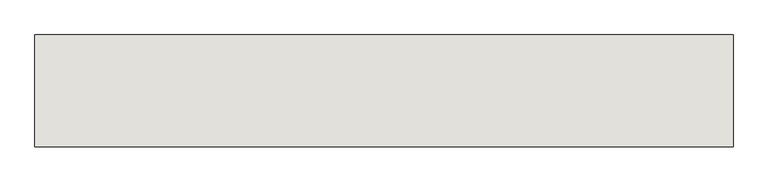
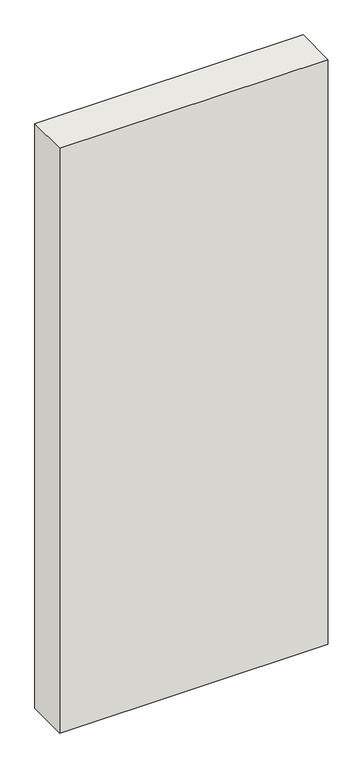
"""IFC4 building model written with IfcOpenShell, lengths in millimetres: wall geometry, Holzwand."""

import ifcopenshell
import ifcopenshell.guid

model = None  # the IFC model being written
_history = None  # IfcOwnerHistory: only IFC2X3 demands one
_inside = {}  # id of a spatial element -> (the spatial element, [elements in it])
_under = {}  # id of a project, library or spatial element -> (it, [spatial elements below it])
_declared = {}  # id of a project -> (the project, [libraries it declares])
_typed = {}  # id of a type object -> (the type object, [elements of that type])
_made_of = {}  # id of a material, layer set ... -> (it, [elements and type objects made of it])


def new_model(schema):
    """Start an empty IFC model of exactly this schema.

    Asked for "IFC4X3", IfcOpenShell would pick the latest addendum, in which some entities
    have other attributes; the version numbers below select the first issue.
    IFC2X3 requires an IfcOwnerHistory on every rooted entity: one is made here for all.
    """
    global model, _history
    if schema == "IFC4X3":
        model = ifcopenshell.file(schema_version=(4, 3, 0, 0))
    else:
        model = ifcopenshell.file(schema=schema)
    _inside.clear()
    _under.clear()
    _declared.clear()
    _typed.clear()
    _made_of.clear()
    _history = None
    if model.schema == "IFC2X3":
        org = make("IfcOrganization", Name="unknown")
        user = make(
            "IfcPersonAndOrganization",
            ThePerson=make("IfcPerson", FamilyName="unknown"),
            TheOrganization=org,
        )
        app = make(
            "IfcApplication",
            ApplicationDeveloper=org,
            Version="unknown",
            ApplicationFullName="unknown",
            ApplicationIdentifier="unknown",
        )
        _history = make(
            "IfcOwnerHistory",
            OwningUser=user,
            OwningApplication=app,
            ChangeAction="ADDED",
            CreationDate=0,
        )
    return model


def make(cls, **values):
    """One entity of the class cls with the attributes given. An attribute that is None is left unset."""
    return model.create_entity(
        cls, **{name: value for name, value in values.items() if value is not None}
    )


def rooted(cls, **values):
    """An entity with a GlobalId (a new one), such as an element, a storey or a relation."""
    return make(cls, GlobalId=ifcopenshell.guid.new(), OwnerHistory=_history, **values)


def si_unit(unit_type, name, prefix=None):
    """IfcSIUnit, for example si_unit("LENGTHUNIT", "METRE", prefix="MILLI")."""
    return make("IfcSIUnit", UnitType=unit_type, Prefix=prefix, Name=name)


def assignment(units):
    """IfcUnitAssignment: the units of a project."""
    return None if units is None else make("IfcUnitAssignment", Units=units)


def point(xyz):
    """IfcCartesianPoint."""
    return None if xyz is None else make("IfcCartesianPoint", Coordinates=xyz)


def direction(xyz):
    """IfcDirection."""
    return None if xyz is None else make("IfcDirection", DirectionRatios=xyz)


def frame(location, z_axis=None, x_axis=None):
    """IfcAxis2Placement3D, a coordinate frame: its origin and axes. An axis left out is left unset."""
    return make(
        "IfcAxis2Placement3D",
        Location=point(location),
        Axis=direction(z_axis),
        RefDirection=direction(x_axis),
    )


def origin():
    """The frame at (0, 0, 0) with its axes left unset."""
    return frame((0.0, 0.0, 0.0))


def origin_with_axes():
    """The frame at (0, 0, 0) with the z axis (0, 0, 1) and the x axis (1, 0, 0) written out."""
    return frame((0.0, 0.0, 0.0), z_axis=(0.0, 0.0, 1.0), x_axis=(1.0, 0.0, 0.0))


def place(relative_to, where):
    """IfcLocalPlacement: puts the frame where relative to a parent placement (None: the world)."""
    return make(
        "IfcLocalPlacement", PlacementRelTo=relative_to, RelativePlacement=where
    )


def context(
    kind, dimensions, precision=None, world=None, true_north=None, identifier=None
):
    """IfcGeometricRepresentationContext, for example the 3D "Model" context."""
    return make(
        "IfcGeometricRepresentationContext",
        ContextIdentifier=identifier,
        ContextType=kind,
        CoordinateSpaceDimension=dimensions,
        Precision=precision,
        WorldCoordinateSystem=world,
        TrueNorth=true_north,
    )


def project(units=None, contexts=None):
    """IfcProject with its units and contexts."""
    return rooted(
        "IfcProject",
        Name="project",
        RepresentationContexts=contexts,
        UnitsInContext=assignment(units),
    )


def spatial(cls, under=None, at=None, **own):
    """A site, building, storey or space (cls), placed at a placement, below another one or the project."""
    s = rooted(cls, ObjectPlacement=at, **own)
    if under is not None:
        _under.setdefault(under.id(), (under, []))[1].append(s)
    return s


def polyline(points):
    """IfcPolyline through the points."""
    return make("IfcPolyline", Points=[point(p) for p in points])


def outline(outer, holes=None, kind="AREA"):
    """IfcArbitraryClosedProfileDef: a profile drawn as a closed curve; with holes, ...WithVoids."""
    if holes is None:
        return make("IfcArbitraryClosedProfileDef", ProfileType=kind, OuterCurve=outer)
    return make(
        "IfcArbitraryProfileDefWithVoids",
        ProfileType=kind,
        OuterCurve=outer,
        InnerCurves=holes,
    )


def extrude(swept, where, along, depth):
    """IfcExtrudedAreaSolid: the profile swept, set in the frame where, extruded along a direction by depth."""
    return make(
        "IfcExtrudedAreaSolid",
        SweptArea=swept,
        Position=where,
        ExtrudedDirection=direction(along),
        Depth=depth,
    )


def shape(context_of_items, identifier, shape_type, items):
    """IfcShapeRepresentation: the items that make up one representation, for example the "Body"."""
    return make(
        "IfcShapeRepresentation",
        ContextOfItems=context_of_items,
        RepresentationIdentifier=identifier,
        RepresentationType=shape_type,
        Items=items,
    )


def source(mapping_origin, context_of_items, identifier, shape_type, items):
    """IfcRepresentationMap: a shape defined once, which mapped items show again and again."""
    return make(
        "IfcRepresentationMap",
        MappingOrigin=mapping_origin,
        MappedRepresentation=shape(context_of_items, identifier, shape_type, items),
    )


def transform(
    local_origin,
    x_axis=None,
    y_axis=None,
    z_axis=None,
    scale=None,
    scale2=None,
    scale3=None,
    uniform=True,
):
    """IfcCartesianTransformationOperator3D, or its non-uniform kind. x_axis, y_axis, z_axis: its Axis1, 2, 3."""
    if uniform:
        return make(
            "IfcCartesianTransformationOperator3D",
            Axis1=direction(x_axis),
            Axis2=direction(y_axis),
            LocalOrigin=point(local_origin),
            Scale=scale,
            Axis3=direction(z_axis),
        )
    return make(
        "IfcCartesianTransformationOperator3DnonUniform",
        Axis1=direction(x_axis),
        Axis2=direction(y_axis),
        LocalOrigin=point(local_origin),
        Scale=scale,
        Axis3=direction(z_axis),
        Scale2=scale2,
        Scale3=scale3,
    )


def mapped(mapping_source, mapping_target):
    """IfcMappedItem: shows the shape of a source again, moved by a transform."""
    return make(
        "IfcMappedItem", MappingSource=mapping_source, MappingTarget=mapping_target
    )


def made_of(thing, what):
    """Note that an element or type object is made of a material, layer set ...; save() writes the relation."""
    if what is not None:
        _made_of.setdefault(what.id(), (what, []))[1].append(thing)
    return thing


def element(
    cls,
    number,
    at=None,
    inside=None,
    cuts=None,
    type_object=None,
    material=None,
    context=None,
    identifier="Body",
    shape_type=None,
    held_by="IfcProductDefinitionShape",
    body=None,
    shapes=None,
    **own,
):
    """One element of the class cls, such as IfcWall. Its Tag is "e" and its number.

    at: its placement. inside: the storey or other place that contains it. cuts: it is an
    opening in that element (IfcRelVoidsElement). A single representation is given by context,
    identifier, shape_type and body (its items); several are given by shapes. held_by: the class
    of the entity that holds the representations. save() writes the other relations.
    """
    e = rooted(cls, Tag="e%d" % number, ObjectPlacement=at, **own)
    if body is not None:
        shapes = [shape(context, identifier, shape_type, body)]
    if shapes is not None:
        e.Representation = make(held_by, Representations=shapes)
    if inside is not None:
        _inside.setdefault(inside.id(), (inside, []))[1].append(e)
    if cuts is not None:
        rooted(
            "IfcRelVoidsElement", RelatingBuildingElement=cuts, RelatedOpeningElement=e
        )
    if type_object is not None:
        _typed.setdefault(type_object.id(), (type_object, []))[1].append(e)
    return made_of(e, material)


def aggregate(whole, parts):
    """IfcRelAggregates: a whole, such as a stair, and the parts it consists of."""
    return rooted("IfcRelAggregates", RelatingObject=whole, RelatedObjects=parts)


def save(model, path):
    """Write the relations noted so far, then the file.

    IfcRelAggregates (storeys below a building ...), IfcRelContainedInSpatialStructure (elements
    in a storey), IfcRelDefinesByType, IfcRelAssociatesMaterial and IfcRelDeclares: one each for
    every whole, place, type object, material and project.
    """
    for whole, parts in _under.values():
        aggregate(whole, parts)
    for where, things in _inside.values():
        rooted(
            "IfcRelContainedInSpatialStructure",
            RelatedElements=things,
            RelatingStructure=where,
        )
    for kind, things in _typed.values():
        rooted("IfcRelDefinesByType", RelatedObjects=things, RelatingType=kind)
    for what, things in _made_of.values():
        rooted("IfcRelAssociatesMaterial", RelatedObjects=things, RelatingMaterial=what)
    for by, libraries in _declared.values():
        rooted("IfcRelDeclares", RelatingContext=by, RelatedDefinitions=libraries)
    model.write(path)


def wall_0f97e130(model_context):
    return source(origin(), model_context, "Body", "SweptSolid", [
        extrude(outline(polyline([(1250.0, 200.0), (1250.0, 0.0), (0.0, 0.0), (0.0, 200.0), (1250.0, 200.0)])), origin_with_axes(), (0.0, 0.0, 1.0), 2880.0),
    ])


if __name__ == "__main__":
    model = new_model("IFC4")
    model_context = context("Model", 3, world=origin())
    ifc_project = project(units=[si_unit("LENGTHUNIT", "METRE", prefix="MILLI")], contexts=[model_context])
    site = spatial("IfcSite", under=ifc_project)
    building = spatial("IfcBuilding", under=site)
    placement = place(None, origin())
    wall_shape = wall_0f97e130(model_context)
    element("IfcWall", 1, ObjectType="Holzwand", at=placement, inside=building, context=model_context, shape_type="MappedRepresentation", body=[
        mapped(wall_shape, transform((0.0, 0.0, 0.0), x_axis=(1.0, 0.0, 0.0), y_axis=(0.0, 1.0, 0.0), z_axis=(0.0, 0.0, 1.0))),
    ])
    save(model, "model.ifc")

# Revit data of these elements
# Element 1 (IfcWall, "Holzwand")
#   Materials on its faces: "holzschalung"
# Materials
#   "holzschalung": class "Unassigned", colour RGB 128 128 128, transparency 0
